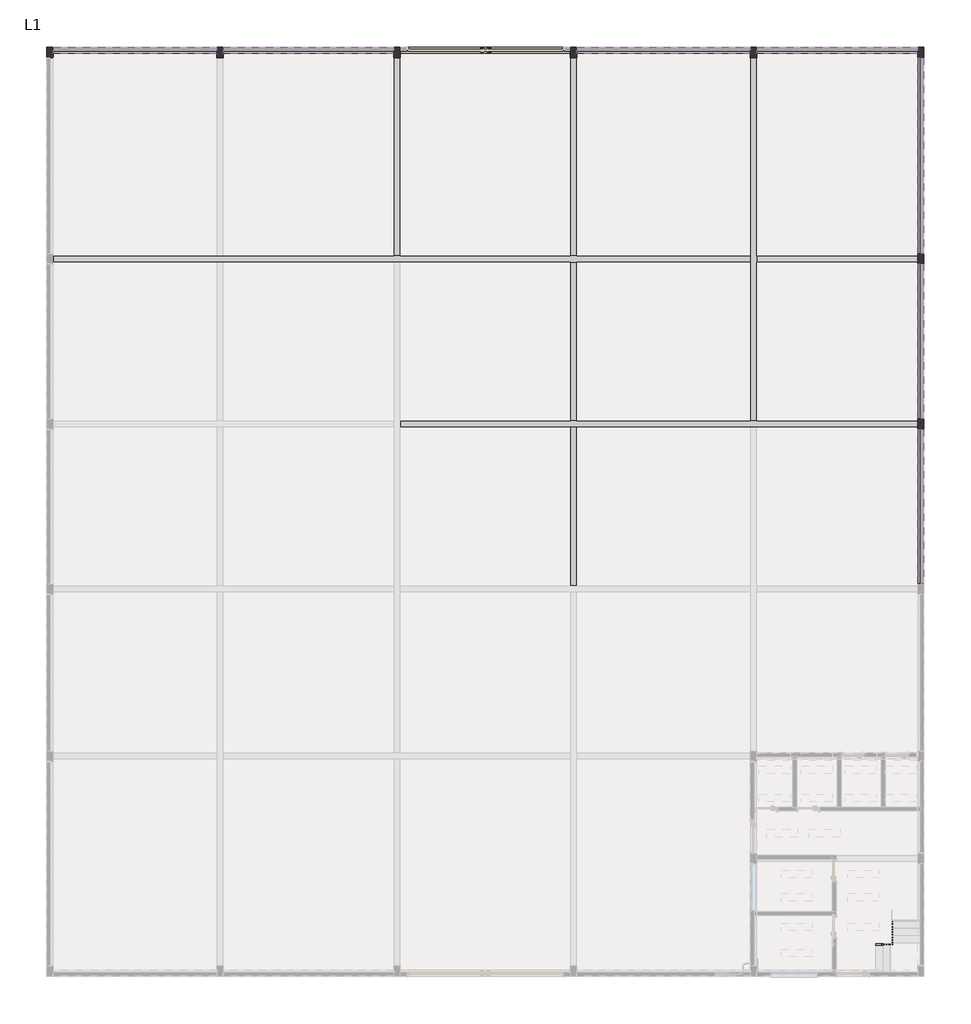
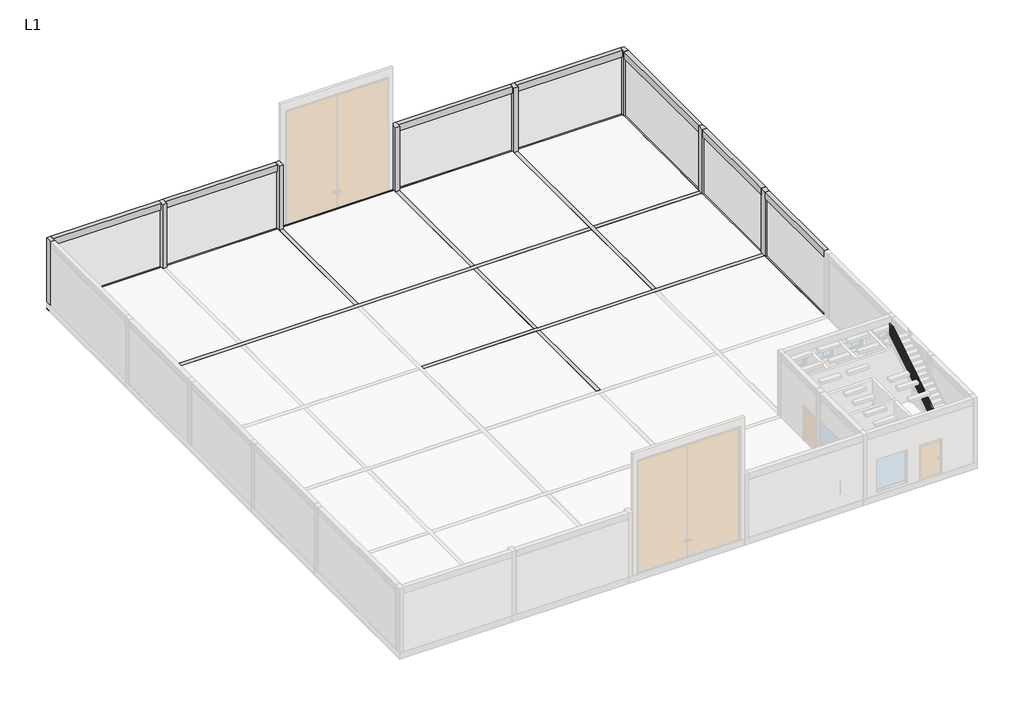
# One storey, part 3 of 4: 23 beams, 8 columns, 1 railing.
"""IFC4 building model written with IfcOpenShell, lengths in millimetres."""

from ifc_helpers import new_model, si_unit, frame, origin, place, context, project, spatial, polyline, outline, extrude, faceted_brep, element, save

model = new_model("IFC4")

# Units and contexts
model_context = context("Model", 3, world=origin())
ifc_project = project(units=[si_unit("LENGTHUNIT", "METRE", prefix="MILLI")], contexts=[model_context])

# Site, building, storey
site = spatial("IfcSite", under=ifc_project)
building = spatial("IfcBuilding", under=site)
storey = spatial("IfcBuildingStorey", under=building, Name="L1", Elevation=0.0)

# Beams
placement = place(None, origin())
element("IfcBeam", 1, ObjectType="M_Hormigón-Viga rectangular : 250 x 400mm", at=placement, inside=storey, context=model_context, shape_type="Brep", body=[
    faceted_brep([(10275.0, 18000.0, 0.0), (10275.0, 17750.0, 0.0), (10525.0, 17750.0, 0.0), (16750.0, 17750.0, 0.0), (17000.0, 17750.0, 0.0), (17000.0, 18000.0, 0.0), (10275.0, 18000.0, -400.0), (17000.0, 18000.0, -400.0), (10275.0, 17750.0, -400.0), (17000.0, 17750.0, -400.0), (16750.0, 17750.0, -400.0), (10525.0, 17750.0, -400.0)], [[[0, 1, 2, 3, 4, 5]], [[6, 0, 5, 7]], [[8, 6, 7, 9, 10, 11]], [[1, 8, 11, 10, 9, 4, 3, 2]], [[1, 0, 6, 8]], [[5, 4, 9, 7]]]),
])
element("IfcBeam", 2, ObjectType="M_Hormigón-Viga rectangular : 250 x 400mm", at=placement, inside=storey, context=model_context, shape_type="Brep", body=[
    faceted_brep([(3300.0, 18000.0, 0.0), (3300.0, 17750.0, 0.0), (3550.0, 17750.0, 0.0), (10275.0, 17750.0, 0.0), (10275.0, 18000.0, 0.0), (3300.0, 18000.0, -400.0), (10275.0, 18000.0, -400.0), (3300.0, 17750.0, -400.0), (10275.0, 17750.0, -400.0), (3550.0, 17750.0, -400.0), (10275.0, 17750.0, -350.0)], [[[0, 1, 2, 3, 4]], [[5, 0, 4, 6]], [[7, 5, 6, 8, 9]], [[1, 7, 9, 8, 10, 3, 2]], [[1, 0, 5, 7]], [[4, 3, 10, 8, 6]]]),
])
element("IfcBeam", 3, ObjectType="M_Hormigón-Viga rectangular : 250 x 400mm", at=placement, inside=storey, context=model_context, shape_type="Brep", body=[
    faceted_brep([(-3550.0, 18000.0, 0.0), (-3550.0, 17750.0, 0.0), (-3300.0, 17750.0, 0.0), (3300.0, 17750.0, 0.0), (3300.0, 18000.0, 0.0), (-3550.0, 18000.0, -400.0), (3300.0, 18000.0, -400.0), (-3550.0, 17750.0, -400.0), (3300.0, 17750.0, -400.0), (-3300.0, 17750.0, -400.0), (3300.0, 17750.0, -350.0)], [[[0, 1, 2, 3, 4]], [[5, 0, 4, 6]], [[7, 5, 6, 8, 9]], [[1, 7, 9, 8, 10, 3, 2]], [[1, 0, 5, 7]], [[4, 3, 10, 8, 6]]]),
])
element("IfcBeam", 4, ObjectType="M_Hormigón-Viga rectangular : 250 x 400mm", at=placement, inside=storey, context=model_context, shape_type="Brep", body=[
    faceted_brep([(-10400.0, 18000.0, 0.0), (-10400.0, 17750.0, 0.0), (-10150.0, 17750.0, 0.0), (-3550.0, 17750.0, 0.0), (-3550.0, 18000.0, 0.0), (-10400.0, 18000.0, -400.0), (-3550.0, 18000.0, -400.0), (-10400.0, 17750.0, -400.0), (-3550.0, 17750.0, -400.0), (-10150.0, 17750.0, -400.0), (-3550.0, 17750.0, -350.0)], [[[0, 1, 2, 3, 4]], [[5, 0, 4, 6]], [[7, 5, 6, 8, 9]], [[1, 7, 9, 8, 10, 3, 2]], [[1, 0, 5, 7]], [[4, 3, 10, 8, 6]]]),
])
element("IfcBeam", 5, ObjectType="M_Hormigón-Viga rectangular : 250 x 400mm", at=placement, inside=storey, context=model_context, shape_type="Brep", body=[
    faceted_brep([(-17000.0, 18000.0, 0.0), (-17000.0, 17750.0, 0.0), (-16750.0, 17750.0, 0.0), (-10400.0, 17750.0, 0.0), (-10400.0, 18000.0, 0.0), (-16750.0, 18000.0, 0.0), (-17000.0, 18000.0, -400.0), (-17000.0, 18000.0, -350.0), (-10400.0, 18000.0, -400.0), (-17000.0, 17750.0, -400.0), (-10400.0, 17750.0, -400.0), (-16750.0, 17750.0, -400.0), (-10400.0, 17750.0, -350.0)], [[[0, 1, 2, 3, 4, 5]], [[6, 7, 0, 5, 4, 8]], [[9, 6, 8, 10, 11]], [[1, 9, 11, 10, 12, 3, 2]], [[1, 0, 7, 6, 9]], [[4, 3, 12, 10, 8]]]),
])
element("IfcBeam", 6, ObjectType="M_Hormigón-Viga rectangular : 250 x 400mm", at=placement, inside=storey, context=model_context, shape_type="Brep", body=[
    faceted_brep([(17000.0, 9675.0, 0.0), (17000.0, 9925.0, 0.0), (16750.0, 9925.0, 0.0), (10525.0, 9925.0, 0.0), (10525.0, 9675.0, 0.0), (16750.0, 9675.0, 0.0), (17000.0, 9925.0, -400.0), (16750.0, 9925.0, -400.0), (10525.0, 9925.0, -400.0), (10525.0, 9925.0, -350.0), (17000.0, 9675.0, -400.0), (16750.0, 9675.0, -400.0), (10525.0, 9675.0, -400.0), (10525.0, 9675.0, -350.0)], [[[0, 1, 2, 3, 4, 5]], [[1, 6, 7, 8, 9, 3, 2]], [[6, 10, 11, 12, 8, 7]], [[10, 0, 5, 4, 13, 12, 11]], [[1, 0, 10, 6]], [[4, 3, 9, 8, 12, 13]]]),
])
element("IfcBeam", 7, ObjectType="M_Hormigón-Viga rectangular : 250 x 400mm", at=placement, inside=storey, context=model_context, shape_type="Brep", body=[
    faceted_brep([(17000.0, 3275.0, 0.0), (17000.0, 3525.0, 0.0), (16750.0, 3525.0, 0.0), (10525.0, 3525.0, 0.0), (10275.0, 3525.0, 0.0), (3550.0, 3525.0, 0.0), (3300.0, 3525.0, 0.0), (-3300.0, 3525.0, 0.0), (-3300.0, 3275.0, 0.0), (3300.0, 3275.0, 0.0), (3550.0, 3275.0, 0.0), (10275.0, 3275.0, 0.0), (10525.0, 3275.0, 0.0), (16750.0, 3275.0, 0.0), (17000.0, 3525.0, -400.0), (16750.0, 3525.0, -400.0), (10525.0, 3525.0, -400.0), (10275.0, 3525.0, -400.0), (3550.0, 3525.0, -400.0), (3300.0, 3525.0, -400.0), (-3300.0, 3525.0, -400.0), (-3300.0, 3525.0, -350.0), (17000.0, 3275.0, -400.0), (16750.0, 3275.0, -400.0), (10525.0, 3275.0, -400.0), (10275.0, 3275.0, -400.0), (3550.0, 3275.0, -400.0), (3300.0, 3275.0, -400.0), (-3300.0, 3275.0, -400.0), (-3300.0, 3275.0, -350.0)], [[[0, 1, 2, 3, 4, 5, 6, 7, 8, 9, 10, 11, 12, 13]], [[1, 14, 15, 16, 17, 18, 19, 20, 21, 7, 6, 5, 4, 3, 2]], [[14, 22, 23, 24, 25, 26, 27, 28, 20, 19, 18, 17, 16, 15]], [[22, 0, 13, 12, 11, 10, 9, 8, 29, 28, 27, 26, 25, 24, 23]], [[1, 0, 22, 14]], [[8, 7, 21, 20, 28, 29]]]),
])
element("IfcBeam", 8, ObjectType="M_Hormigón-Viga rectangular : 250 x 400mm", at=placement, inside=storey, context=model_context, shape_type="Brep", body=[
    faceted_brep([(17000.0, 3275.0, 0.0), (16750.0, 3275.0, 0.0), (16750.0, 3200.0, 0.0), (16750.0, -2800.0, 0.0), (16750.0, -2875.0, 0.0), (17000.0, -2875.0, 0.0), (17000.0, -2800.0, 0.0), (17000.0, 3200.0, 0.0), (17000.0, 3275.0, -400.0), (17000.0, -2875.0, -400.0), (16750.0, 3275.0, -400.0), (16750.0, -2875.0, -400.0), (16750.0, 3275.0, -350.0), (16750.0, -2875.0, -350.0)], [[[0, 1, 2, 3, 4, 5, 6, 7]], [[8, 0, 7, 6, 5, 9]], [[10, 8, 9, 11]], [[1, 12, 10, 11, 13, 4, 3, 2]], [[1, 0, 8, 10, 12]], [[5, 4, 13, 11, 9]]]),
])
element("IfcBeam", 9, ObjectType="M_Hormigón-Viga rectangular : 250 x 400mm", at=placement, inside=storey, context=model_context, shape_type="Brep", body=[
    faceted_brep([(17000.0, 9675.0, 0.0), (16750.0, 9675.0, 0.0), (16750.0, 9600.0, 0.0), (16750.0, 3600.0, 0.0), (16750.0, 3525.0, 0.0), (17000.0, 3525.0, 0.0), (17000.0, 3600.0, 0.0), (17000.0, 9600.0, 0.0), (17000.0, 9675.0, -400.0), (17000.0, 3525.0, -400.0), (16750.0, 9675.0, -400.0), (16750.0, 3525.0, -400.0), (16750.0, 9675.0, -350.0), (16750.0, 3525.0, -350.0)], [[[0, 1, 2, 3, 4, 5, 6, 7]], [[8, 0, 7, 6, 5, 9]], [[10, 8, 9, 11]], [[1, 12, 10, 11, 13, 4, 3, 2]], [[1, 0, 8, 10, 12]], [[5, 4, 13, 11, 9]]]),
])
element("IfcBeam", 10, ObjectType="M_Hormigón-Viga rectangular : 250 x 400mm", at=placement, inside=storey, context=model_context, shape_type="Brep", body=[
    faceted_brep([(16750.0, 9925.0, 0.0), (17000.0, 9925.0, 0.0), (17000.0, 10000.0, 0.0), (17000.0, 17600.0, 0.0), (17000.0, 17750.0, 0.0), (16750.0, 17750.0, 0.0), (16750.0, 17600.0, 0.0), (16750.0, 10000.0, 0.0), (17000.0, 9925.0, -400.0), (17000.0, 17750.0, -400.0), (16750.0, 9925.0, -400.0), (16750.0, 17750.0, -400.0), (16750.0, 9925.0, -350.0), (16750.0, 17750.0, -350.0)], [[[0, 1, 2, 3, 4, 5, 6, 7]], [[1, 8, 9, 4, 3, 2]], [[8, 10, 11, 9]], [[10, 12, 0, 7, 6, 5, 13, 11]], [[1, 0, 12, 10, 8]], [[5, 4, 9, 11, 13]]]),
])
element("IfcBeam", 11, ObjectType="M_Hormigón-Viga rectangular : 250 x 400mm", at=placement, inside=storey, context=model_context, shape_type="Brep", body=[
    faceted_brep([(-3300.0, 17750.0, 0.0), (-3550.0, 17750.0, 0.0), (-3550.0, 9925.0, 0.0), (-3300.0, 9925.0, 0.0), (-3300.0, 17750.0, -400.0), (-3300.0, 17750.0, -350.0), (-3300.0, 9925.0, -350.0), (-3300.0, 9925.0, -400.0), (-3550.0, 17750.0, -400.0), (-3550.0, 9925.0, -400.0), (-3550.0, 17750.0, -350.0), (-3550.0, 9925.0, -350.0)], [[[0, 1, 2, 3]], [[4, 5, 0, 3, 6, 7]], [[8, 4, 7, 9]], [[1, 10, 8, 9, 11, 2]], [[1, 0, 5, 4, 8, 10]], [[3, 2, 11, 9, 7, 6]]]),
])
element("IfcBeam", 12, ObjectType="M_Hormigón-Viga rectangular : 250 x 400mm", at=placement, inside=storey, context=model_context, shape_type="Brep", body=[
    faceted_brep([(3550.0, 17750.0, 0.0), (3300.0, 17750.0, 0.0), (3300.0, 9925.0, 0.0), (3550.0, 9925.0, 0.0), (3550.0, 17750.0, -400.0), (3550.0, 17750.0, -350.0), (3550.0, 9925.0, -350.0), (3550.0, 9925.0, -400.0), (3300.0, 17750.0, -400.0), (3300.0, 9925.0, -400.0), (3300.0, 17750.0, -350.0), (3300.0, 9925.0, -350.0)], [[[0, 1, 2, 3]], [[4, 5, 0, 3, 6, 7]], [[8, 4, 7, 9]], [[1, 10, 8, 9, 11, 2]], [[1, 0, 5, 4, 8, 10]], [[3, 2, 11, 9, 7, 6]]]),
])
element("IfcBeam", 13, ObjectType="M_Hormigón-Viga rectangular : 250 x 400mm", at=placement, inside=storey, context=model_context, shape_type="Brep", body=[
    faceted_brep([(-16750.0, 9925.0, 0.0), (-16750.0, 9675.0, 0.0), (-10400.0, 9675.0, 0.0), (-10150.0, 9675.0, 0.0), (-3550.0, 9675.0, 0.0), (-3300.0, 9675.0, 0.0), (3300.0, 9675.0, 0.0), (3550.0, 9675.0, 0.0), (10275.0, 9675.0, 0.0), (10275.0, 9925.0, 0.0), (3550.0, 9925.0, 0.0), (3300.0, 9925.0, 0.0), (-3300.0, 9925.0, 0.0), (-3550.0, 9925.0, 0.0), (-10150.0, 9925.0, 0.0), (-10400.0, 9925.0, 0.0), (-16750.0, 9925.0, -400.0), (-16750.0, 9925.0, -350.0), (10275.0, 9925.0, -350.0), (10275.0, 9925.0, -400.0), (3550.0, 9925.0, -400.0), (3300.0, 9925.0, -400.0), (-3300.0, 9925.0, -400.0), (-3550.0, 9925.0, -400.0), (-10150.0, 9925.0, -400.0), (-10400.0, 9925.0, -400.0), (-16750.0, 9675.0, -400.0), (10275.0, 9675.0, -400.0), (3550.0, 9675.0, -400.0), (3300.0, 9675.0, -400.0), (-3300.0, 9675.0, -400.0), (-3550.0, 9675.0, -400.0), (-10150.0, 9675.0, -400.0), (-10400.0, 9675.0, -400.0), (-16750.0, 9675.0, -350.0), (10275.0, 9675.0, -350.0)], [[[0, 1, 2, 3, 4, 5, 6, 7, 8, 9, 10, 11, 12, 13, 14, 15]], [[16, 17, 0, 15, 14, 13, 12, 11, 10, 9, 18, 19, 20, 21, 22, 23, 24, 25]], [[26, 16, 25, 24, 23, 22, 21, 20, 19, 27, 28, 29, 30, 31, 32, 33]], [[1, 34, 26, 33, 32, 31, 30, 29, 28, 27, 35, 8, 7, 6, 5, 4, 3, 2]], [[1, 0, 17, 16, 26, 34]], [[9, 8, 35, 27, 19, 18]]]),
])
element("IfcBeam", 14, ObjectType="M_Hormigón-Viga rectangular : 250 x 400mm", at=placement, inside=storey, context=model_context, shape_type="Brep", body=[
    faceted_brep([(3550.0, 9675.0, 0.0), (3300.0, 9675.0, 0.0), (3300.0, 3525.0, 0.0), (3550.0, 3525.0, 0.0), (3550.0, 9675.0, -400.0), (3550.0, 9675.0, -350.0), (3550.0, 3525.0, -350.0), (3550.0, 3525.0, -400.0), (3300.0, 9675.0, -400.0), (3300.0, 3525.0, -400.0), (3300.0, 9675.0, -350.0), (3300.0, 3525.0, -350.0)], [[[0, 1, 2, 3]], [[4, 5, 0, 3, 6, 7]], [[8, 4, 7, 9]], [[1, 10, 8, 9, 11, 2]], [[1, 0, 5, 4, 8, 10]], [[3, 2, 11, 9, 7, 6]]]),
])
element("IfcBeam", 15, ObjectType="M_Hormigón-Viga rectangular : 250 x 400mm", at=placement, inside=storey, context=model_context, shape_type="Brep", body=[
    faceted_brep([(10525.0, 17750.0, 0.0), (10275.0, 17750.0, 0.0), (10275.0, 9925.0, 0.0), (10275.0, 9675.0, 0.0), (10275.0, 3525.0, 0.0), (10525.0, 3525.0, 0.0), (10525.0, 9675.0, 0.0), (10525.0, 9925.0, 0.0), (10525.0, 17750.0, -400.0), (10525.0, 17750.0, -350.0), (10525.0, 3525.0, -350.0), (10525.0, 3525.0, -400.0), (10525.0, 9675.0, -400.0), (10525.0, 9925.0, -400.0), (10275.0, 17750.0, -400.0), (10275.0, 3525.0, -400.0), (10275.0, 9675.0, -400.0), (10275.0, 9925.0, -400.0), (10275.0, 17750.0, -350.0), (10275.0, 3525.0, -350.0)], [[[0, 1, 2, 3, 4, 5, 6, 7]], [[8, 9, 0, 7, 6, 5, 10, 11, 12, 13]], [[14, 8, 13, 12, 11, 15, 16, 17]], [[1, 18, 14, 17, 16, 15, 19, 4, 3, 2]], [[1, 0, 9, 8, 14, 18]], [[5, 4, 19, 15, 11, 10]]]),
])
element("IfcBeam", 16, ObjectType="M_Hormigón-Viga rectangular : 250 x 400mm", at=placement, inside=storey, context=model_context, shape_type="Brep", body=[
    faceted_brep([(3550.0, 3275.0, 0.0), (3300.0, 3275.0, 0.0), (3300.0, -2875.0, 0.0), (3550.0, -2875.0, 0.0), (3550.0, 3275.0, -400.0), (3550.0, 3275.0, -350.0), (3550.0, -2875.0, -350.0), (3550.0, -2875.0, -400.0), (3300.0, 3275.0, -400.0), (3300.0, -2875.0, -400.0), (3300.0, 3275.0, -350.0), (3300.0, -2875.0, -350.0)], [[[0, 1, 2, 3]], [[4, 5, 0, 3, 6, 7]], [[8, 4, 7, 9]], [[1, 10, 8, 9, 11, 2]], [[1, 0, 5, 4, 8, 10]], [[3, 2, 11, 9, 7, 6]]]),
])
element("IfcBeam", 17, ObjectType="M_Hormigón-Viga rectangular : 250 x 400mm", at=placement, inside=storey, context=model_context, shape_type="SweptSolid", body=[
    extrude(outline(polyline([(10525.0, 17750.0), (10525.0, 18000.0), (16750.0, 18000.0), (16750.0, 17750.0), (10525.0, 17750.0)])), frame((0.0, 0.0, 3600.0), z_axis=(0.0, 0.0, 1.0), x_axis=(1.0, 0.0, 0.0)), (0.0, 0.0, 1.0), 400.0),
])
element("IfcBeam", 18, ObjectType="M_Hormigón-Viga rectangular : 250 x 400mm", at=placement, inside=storey, context=model_context, shape_type="SweptSolid", body=[
    extrude(outline(polyline([(3550.0, 17750.0), (3550.0, 18000.0), (10275.0, 18000.0), (10275.0, 17750.0), (3550.0, 17750.0)])), frame((0.0, 0.0, 3600.0), z_axis=(0.0, 0.0, 1.0), x_axis=(1.0, 0.0, 0.0)), (0.0, 0.0, 1.0), 400.0),
])
element("IfcBeam", 19, ObjectType="M_Hormigón-Viga rectangular : 250 x 400mm", at=placement, inside=storey, context=model_context, shape_type="SweptSolid", body=[
    extrude(outline(polyline([(-3550.0, 18000.0), (-3550.0, 17750.0), (-10150.0, 17750.0), (-10150.0, 18000.0), (-3550.0, 18000.0)])), frame((0.0, 0.0, 3600.0), z_axis=(0.0, 0.0, 1.0), x_axis=(1.0, 0.0, 0.0)), (0.0, 0.0, 1.0), 400.0),
])
element("IfcBeam", 20, ObjectType="M_Hormigón-Viga rectangular : 250 x 400mm", at=placement, inside=storey, context=model_context, shape_type="SweptSolid", body=[
    extrude(outline(polyline([(-16750.0, 17750.0), (-16750.0, 18000.0), (-10400.0, 18000.0), (-10400.0, 17750.0), (-16750.0, 17750.0)])), frame((0.0, 0.0, 3600.0), z_axis=(0.0, 0.0, 1.0), x_axis=(1.0, 0.0, 0.0)), (0.0, 0.0, 1.0), 400.0),
])
element("IfcBeam", 21, ObjectType="M_Hormigón-Viga rectangular : 250 x 400mm", at=placement, inside=storey, context=model_context, shape_type="SweptSolid", body=[
    extrude(outline(polyline([(16750.0, 3200.0), (17000.0, 3200.0), (17000.0, -2800.0), (16750.0, -2800.0), (16750.0, 3200.0)])), frame((0.0, 0.0, 3600.0), z_axis=(0.0, 0.0, 1.0), x_axis=(1.0, 0.0, 0.0)), (0.0, 0.0, 1.0), 400.0),
])
element("IfcBeam", 22, ObjectType="M_Hormigón-Viga rectangular : 250 x 400mm", at=placement, inside=storey, context=model_context, shape_type="SweptSolid", body=[
    extrude(outline(polyline([(16750.0, 9600.0), (17000.0, 9600.0), (17000.0, 3600.0), (16750.0, 3600.0), (16750.0, 9600.0)])), frame((0.0, 0.0, 3600.0), z_axis=(0.0, 0.0, 1.0), x_axis=(1.0, 0.0, 0.0)), (0.0, 0.0, 1.0), 400.0),
])
element("IfcBeam", 23, ObjectType="M_Hormigón-Viga rectangular : 250 x 400mm", at=placement, inside=storey, context=model_context, shape_type="SweptSolid", body=[
    extrude(outline(polyline([(16750.0, 17600.0), (17000.0, 17600.0), (17000.0, 10000.0), (16750.0, 10000.0), (16750.0, 17600.0)])), frame((0.0, 0.0, 3600.0), z_axis=(0.0, 0.0, 1.0), x_axis=(1.0, 0.0, 0.0)), (0.0, 0.0, 1.0), 400.0),
])

# Columns
element("IfcColumn", 24, ObjectType="M_Hormigón-Rectangular-Pilar : 250 x 400mm", at=placement, inside=storey, context=model_context, shape_type="Brep", body=[
    faceted_brep([(-17000.0, 17600.0, 0.0), (-17000.0, 17750.0, 0.0), (-17000.0, 18000.0, 0.0), (-16750.0, 18000.0, 0.0), (-16750.0, 17750.0, 0.0), (-16750.0, 17600.0, 0.0), (-17000.0, 17600.0, 4000.0), (-17000.0, 18000.0, 4000.0), (-16750.0, 18000.0, 4000.0), (-16750.0, 17600.0, 4000.0)], [[[0, 1, 2, 3, 4, 5]], [[6, 7, 2, 1, 0]], [[7, 8, 3, 2]], [[8, 9, 5, 4, 3]], [[9, 6, 0, 5]], [[6, 9, 8, 7]]]),
])
element("IfcColumn", 25, ObjectType="M_Hormigón-Rectangular-Pilar : 250 x 400mm", at=placement, inside=storey, context=model_context, shape_type="Brep", body=[
    faceted_brep([(-3550.0, 17600.0, 0.0), (-3550.0, 17750.0, 0.0), (-3550.0, 18000.0, 0.0), (-3300.0, 18000.0, 0.0), (-3300.0, 17750.0, 0.0), (-3300.0, 17600.0, 0.0), (-3550.0, 17600.0, 4000.0), (-3550.0, 18000.0, 4000.0), (-3300.0, 18000.0, 4000.0), (-3300.0, 17600.0, 4000.0)], [[[0, 1, 2, 3, 4, 5]], [[6, 7, 2, 1, 0]], [[7, 8, 3, 2]], [[8, 9, 5, 4, 3]], [[9, 6, 0, 5]], [[6, 9, 8, 7]]]),
])
element("IfcColumn", 26, ObjectType="M_Hormigón-Rectangular-Pilar : 250 x 400mm", at=placement, inside=storey, context=model_context, shape_type="Brep", body=[
    faceted_brep([(3300.0, 17600.0, 0.0), (3300.0, 17750.0, 0.0), (3300.0, 18000.0, 0.0), (3550.0, 18000.0, 0.0), (3550.0, 17750.0, 0.0), (3550.0, 17600.0, 0.0), (3300.0, 17600.0, 4000.0), (3300.0, 18000.0, 4000.0), (3550.0, 18000.0, 4000.0), (3550.0, 17600.0, 4000.0)], [[[0, 1, 2, 3, 4, 5]], [[6, 7, 2, 1, 0]], [[7, 8, 3, 2]], [[8, 9, 5, 4, 3]], [[9, 6, 0, 5]], [[6, 9, 8, 7]]]),
])
element("IfcColumn", 27, ObjectType="M_Hormigón-Rectangular-Pilar : 250 x 400mm", at=placement, inside=storey, context=model_context, shape_type="Brep", body=[
    faceted_brep([(10275.0, 17600.0, 0.0), (10275.0, 17750.0, 0.0), (10275.0, 18000.0, 0.0), (10525.0, 18000.0, 0.0), (10525.0, 17750.0, 0.0), (10525.0, 17600.0, 0.0), (10275.0, 17600.0, 4000.0), (10275.0, 18000.0, 4000.0), (10525.0, 18000.0, 4000.0), (10525.0, 17600.0, 4000.0)], [[[0, 1, 2, 3, 4, 5]], [[6, 7, 2, 1, 0]], [[7, 8, 3, 2]], [[8, 9, 5, 4, 3]], [[9, 6, 0, 5]], [[6, 9, 8, 7]]]),
])
element("IfcColumn", 28, ObjectType="M_Hormigón-Rectangular-Pilar : 250 x 400mm", at=placement, inside=storey, context=model_context, shape_type="Brep", body=[
    faceted_brep([(16750.0, 17600.0, 0.0), (16750.0, 17750.0, 0.0), (16750.0, 18000.0, 0.0), (17000.0, 18000.0, 0.0), (17000.0, 17750.0, 0.0), (17000.0, 17600.0, 0.0), (16750.0, 17600.0, 4000.0), (16750.0, 18000.0, 4000.0), (17000.0, 18000.0, 4000.0), (17000.0, 17600.0, 4000.0)], [[[0, 1, 2, 3, 4, 5]], [[6, 7, 2, 1, 0]], [[7, 8, 3, 2]], [[8, 9, 5, 4, 3]], [[9, 6, 0, 5]], [[6, 9, 8, 7]]]),
])
element("IfcColumn", 29, ObjectType="M_Hormigón-Rectangular-Pilar : 250 x 400mm", at=placement, inside=storey, context=model_context, shape_type="Brep", body=[
    faceted_brep([(-10400.0, 17600.0, 0.0), (-10400.0, 17750.0, 0.0), (-10400.0, 18000.0, 0.0), (-10150.0, 18000.0, 0.0), (-10150.0, 17750.0, 0.0), (-10150.0, 17600.0, 0.0), (-10400.0, 17600.0, 4000.0), (-10400.0, 18000.0, 4000.0), (-10150.0, 18000.0, 4000.0), (-10150.0, 17600.0, 4000.0)], [[[0, 1, 2, 3, 4, 5]], [[6, 7, 2, 1, 0]], [[7, 8, 3, 2]], [[8, 9, 5, 4, 3]], [[9, 6, 0, 5]], [[6, 9, 8, 7]]]),
])
element("IfcColumn", 30, ObjectType="M_Hormigón-Rectangular-Pilar : 250 x 400mm", at=placement, inside=storey, context=model_context, shape_type="Brep", body=[
    faceted_brep([(16750.0, 9600.0, 0.0), (16750.0, 9675.0, 0.0), (16750.0, 9925.0, 0.0), (16750.0, 10000.0, 0.0), (17000.0, 10000.0, 0.0), (17000.0, 9925.0, 0.0), (17000.0, 9675.0, 0.0), (17000.0, 9600.0, 0.0), (16750.0, 9600.0, 4000.0), (16750.0, 10000.0, 4000.0), (17000.0, 10000.0, 4000.0), (17000.0, 9600.0, 4000.0)], [[[0, 1, 2, 3, 4, 5, 6, 7]], [[8, 9, 3, 2, 1, 0]], [[9, 10, 4, 3]], [[10, 11, 7, 6, 5, 4]], [[11, 8, 0, 7]], [[8, 11, 10, 9]]]),
])
element("IfcColumn", 31, ObjectType="M_Hormigón-Rectangular-Pilar : 250 x 400mm", at=placement, inside=storey, context=model_context, shape_type="Brep", body=[
    faceted_brep([(16750.0, 3200.0, 0.0), (16750.0, 3275.0, 0.0), (16750.0, 3525.0, 0.0), (16750.0, 3600.0, 0.0), (17000.0, 3600.0, 0.0), (17000.0, 3525.0, 0.0), (17000.0, 3275.0, 0.0), (17000.0, 3200.0, 0.0), (16750.0, 3200.0, 4000.0), (16750.0, 3600.0, 4000.0), (17000.0, 3600.0, 4000.0), (17000.0, 3200.0, 4000.0)], [[[0, 1, 2, 3, 4, 5, 6, 7]], [[8, 9, 3, 2, 1, 0]], [[9, 10, 4, 3]], [[10, 11, 7, 6, 5, 4]], [[11, 8, 0, 7]], [[8, 11, 10, 9]]]),
])

# Railing
element("IfcRailing", 32, ObjectType="Pasamanos - Rectangular", at=placement, inside=storey, context=model_context, shape_type="SolidModel", body=[
    faceted_brep([(15137.5726879, -16747.8618478, 1073.9130435), (15137.5726879, -16747.8618478, 1014.753434), (15137.5726879, -16797.8618478, 1014.753434), (15137.5726879, -16797.8618478, 1073.9130435), (15687.5726879, -16747.8618478, 1421.7391304), (15702.0563204, -16747.8618478, 1371.7391304), (15702.0563204, -16797.8618478, 1371.7391304), (15687.5726879, -16797.8618478, 1421.7391304), (15797.9726879, -16747.8618478, 1421.7391304), (15797.9726879, -16797.8618478, 1421.7391304), (15797.9726879, -16797.8618478, 1371.7391304), (15797.9726879, -16747.8618478, 1371.7391304)], [[[0, 1, 2, 3]], [[1, 0, 4, 5]], [[2, 1, 5, 6]], [[3, 2, 6, 7]], [[0, 3, 7, 4]], [[8, 9, 10, 11]], [[5, 4, 8, 11]], [[6, 5, 11, 10]], [[7, 6, 10, 9]], [[4, 7, 9, 8]]]),
    faceted_brep([(15747.9726879, -16747.8618478, 1480.4200194), (15747.9726879, -16747.8618478, 1352.8512657), (15797.9726879, -16747.8618478, 1352.8512657), (15797.9726879, -16747.8618478, 1480.4200194), (15747.9726879, -16698.7691378, 1595.6521739), (15747.9726879, -16658.8763415, 1561.7212103), (15797.9726879, -16658.8763415, 1561.7212103), (15797.9726879, -16698.7691378, 1595.6521739), (15747.9726879, -11473.7691378, 4900.0), (15747.9726879, -11459.2855053, 4850.0), (15797.9726879, -11459.2855053, 4850.0), (15797.9726879, -11473.7691378, 4900.0), (15747.9726879, -11198.7691378, 4900.0), (15797.9726879, -11198.7691378, 4900.0), (15797.9726879, -11198.7691378, 4850.0), (15747.9726879, -11198.7691378, 4850.0)], [[[0, 1, 2, 3]], [[1, 0, 4, 5]], [[2, 1, 5, 6]], [[3, 2, 6, 7]], [[0, 3, 7, 4]], [[5, 4, 8, 9]], [[6, 5, 9, 10]], [[7, 6, 10, 11]], [[4, 7, 11, 8]], [[12, 13, 14, 15]], [[9, 8, 12, 15]], [[10, 9, 15, 14]], [[11, 10, 14, 13]], [[8, 11, 13, 12]]]),
    extrude(outline(polyline([(15762.9726879, -11222.3691378), (15762.9726879, -11202.3691378), (15782.9726879, -11202.3691378), (15782.9726879, -11222.3691378), (15762.9726879, -11222.3691378)])), frame((0.0, 0.0, 4000.0), z_axis=(0.0, 0.0, 1.0), x_axis=(1.0, 0.0, 0.0)), (0.0, 0.0, 1.0), 850.0),
    extrude(outline(polyline([(15762.9726879, -11323.9691378), (15762.9726879, -11303.9691378), (15782.9726879, -11303.9691378), (15782.9726879, -11323.9691378), (15762.9726879, -11323.9691378)])), frame((0.0, 0.0, 4000.0), z_axis=(0.0, 0.0, 1.0), x_axis=(1.0, 0.0, 0.0)), (0.0, 0.0, 1.0), 850.0),
    extrude(outline(polyline([(15762.9726879, -11425.5691378), (15762.9726879, -11405.5691378), (15782.9726879, -11405.5691378), (15782.9726879, -11425.5691378), (15762.9726879, -11425.5691378)])), frame((0.0, 0.0, 4000.0), z_axis=(0.0, 0.0, 1.0), x_axis=(1.0, 0.0, 0.0)), (0.0, 0.0, 1.0), 850.0),
    extrude(outline(polyline([(-11527.1691378, 4807.0696395), (-11507.1691378, 4819.7178609), (-11507.1691378, 3826.0869565), (-11527.1691378, 3826.0869565), (-11527.1691378, 4807.0696395)])), frame((15762.9726879, 0.0, 0.0), z_axis=(1.0, 0.0, 0.0), x_axis=(0.0, 1.0, 0.0)), (0.0, 0.0, 1.0), 20.0),
    extrude(outline(polyline([(-11628.7691378, 4742.8166751), (-11608.7691378, 4755.4648964), (-11608.7691378, 3826.0869565), (-11628.7691378, 3826.0869565), (-11628.7691378, 4742.8166751)])), frame((15762.9726879, 0.0, 0.0), z_axis=(1.0, 0.0, 0.0), x_axis=(0.0, 1.0, 0.0)), (0.0, 0.0, 1.0), 20.0),
    extrude(outline(polyline([(-11730.3691378, 4678.5637107), (-11710.3691378, 4691.211932), (-11710.3691378, 3826.0869565), (-11730.3691378, 3826.0869565), (-11730.3691378, 4678.5637107)])), frame((15762.9726879, 0.0, 0.0), z_axis=(1.0, 0.0, 0.0), x_axis=(0.0, 1.0, 0.0)), (0.0, 0.0, 1.0), 20.0),
    extrude(outline(polyline([(-11831.9691378, 4614.3107462), (-11811.9691378, 4626.9589676), (-11811.9691378, 3652.173913), (-11831.9691378, 3652.173913), (-11831.9691378, 4614.3107462)])), frame((15762.9726879, 0.0, 0.0), z_axis=(1.0, 0.0, 0.0), x_axis=(0.0, 1.0, 0.0)), (0.0, 0.0, 1.0), 20.0),
    extrude(outline(polyline([(-11933.5691378, 4550.0577818), (-11913.5691378, 4562.7060032), (-11913.5691378, 3652.173913), (-11933.5691378, 3652.173913), (-11933.5691378, 4550.0577818)])), frame((15762.9726879, 0.0, 0.0), z_axis=(1.0, 0.0, 0.0), x_axis=(0.0, 1.0, 0.0)), (0.0, 0.0, 1.0), 20.0),
    extrude(outline(polyline([(-12035.1691378, 4485.8048174), (-12015.1691378, 4498.4530387), (-12015.1691378, 3478.2608696), (-12035.1691378, 3478.2608696), (-12035.1691378, 4485.8048174)])), frame((15762.9726879, 0.0, 0.0), z_axis=(1.0, 0.0, 0.0), x_axis=(0.0, 1.0, 0.0)), (0.0, 0.0, 1.0), 20.0),
    extrude(outline(polyline([(-12136.7691378, 4421.551853), (-12116.7691378, 4434.2000743), (-12116.7691378, 3478.2608696), (-12136.7691378, 3478.2608696), (-12136.7691378, 4421.551853)])), frame((15762.9726879, 0.0, 0.0), z_axis=(1.0, 0.0, 0.0), x_axis=(0.0, 1.0, 0.0)), (0.0, 0.0, 1.0), 20.0),
    extrude(outline(polyline([(-12238.3691378, 4357.2988885), (-12218.3691378, 4369.9471099), (-12218.3691378, 3478.2608696), (-12238.3691378, 3478.2608696), (-12238.3691378, 4357.2988885)])), frame((15762.9726879, 0.0, 0.0), z_axis=(1.0, 0.0, 0.0), x_axis=(0.0, 1.0, 0.0)), (0.0, 0.0, 1.0), 20.0),
    extrude(outline(polyline([(-12339.9691378, 4293.0459241), (-12319.9691378, 4305.6941455), (-12319.9691378, 3304.3478261), (-12339.9691378, 3304.3478261), (-12339.9691378, 4293.0459241)])), frame((15762.9726879, 0.0, 0.0), z_axis=(1.0, 0.0, 0.0), x_axis=(0.0, 1.0, 0.0)), (0.0, 0.0, 1.0), 20.0),
    extrude(outline(polyline([(-12441.5691378, 4228.7929597), (-12421.5691378, 4241.441181), (-12421.5691378, 3304.3478261), (-12441.5691378, 3304.3478261), (-12441.5691378, 4228.7929597)])), frame((15762.9726879, 0.0, 0.0), z_axis=(1.0, 0.0, 0.0), x_axis=(0.0, 1.0, 0.0)), (0.0, 0.0, 1.0), 20.0),
    extrude(outline(polyline([(-12543.1691378, 4164.5399953), (-12523.1691378, 4177.1882166), (-12523.1691378, 3304.3478261), (-12543.1691378, 3304.3478261), (-12543.1691378, 4164.5399953)])), frame((15762.9726879, 0.0, 0.0), z_axis=(1.0, 0.0, 0.0), x_axis=(0.0, 1.0, 0.0)), (0.0, 0.0, 1.0), 20.0),
    extrude(outline(polyline([(-12644.7691378, 4100.2870308), (-12624.7691378, 4112.9352522), (-12624.7691378, 3130.4347826), (-12644.7691378, 3130.4347826), (-12644.7691378, 4100.2870308)])), frame((15762.9726879, 0.0, 0.0), z_axis=(1.0, 0.0, 0.0), x_axis=(0.0, 1.0, 0.0)), (0.0, 0.0, 1.0), 20.0),
    extrude(outline(polyline([(-12746.3691378, 4036.0340664), (-12726.3691378, 4048.6822877), (-12726.3691378, 3130.4347826), (-12746.3691378, 3130.4347826), (-12746.3691378, 4036.0340664)])), frame((15762.9726879, 0.0, 0.0), z_axis=(1.0, 0.0, 0.0), x_axis=(0.0, 1.0, 0.0)), (0.0, 0.0, 1.0), 20.0),
    extrude(outline(polyline([(-12847.9691378, 3971.781102), (-12827.9691378, 3984.4293233), (-12827.9691378, 3130.4347826), (-12847.9691378, 3130.4347826), (-12847.9691378, 3971.781102)])), frame((15762.9726879, 0.0, 0.0), z_axis=(1.0, 0.0, 0.0), x_axis=(0.0, 1.0, 0.0)), (0.0, 0.0, 1.0), 20.0),
    extrude(outline(polyline([(-12949.5691378, 3907.5281375), (-12929.5691378, 3920.1763589), (-12929.5691378, 2956.5217391), (-12949.5691378, 2956.5217391), (-12949.5691378, 3907.5281375)])), frame((15762.9726879, 0.0, 0.0), z_axis=(1.0, 0.0, 0.0), x_axis=(0.0, 1.0, 0.0)), (0.0, 0.0, 1.0), 20.0),
    extrude(outline(polyline([(-13051.1691378, 3843.2751731), (-13031.1691378, 3855.9233945), (-13031.1691378, 2956.5217391), (-13051.1691378, 2956.5217391), (-13051.1691378, 3843.2751731)])), frame((15762.9726879, 0.0, 0.0), z_axis=(1.0, 0.0, 0.0), x_axis=(0.0, 1.0, 0.0)), (0.0, 0.0, 1.0), 20.0),
    extrude(outline(polyline([(-13152.7691378, 3779.0222087), (-13132.7691378, 3791.67043), (-13132.7691378, 2782.6086957), (-13152.7691378, 2782.6086957), (-13152.7691378, 3779.0222087)])), frame((15762.9726879, 0.0, 0.0), z_axis=(1.0, 0.0, 0.0), x_axis=(0.0, 1.0, 0.0)), (0.0, 0.0, 1.0), 20.0),
    extrude(outline(polyline([(-13254.3691378, 3714.7692443), (-13234.3691378, 3727.4174656), (-13234.3691378, 2782.6086957), (-13254.3691378, 2782.6086957), (-13254.3691378, 3714.7692443)])), frame((15762.9726879, 0.0, 0.0), z_axis=(1.0, 0.0, 0.0), x_axis=(0.0, 1.0, 0.0)), (0.0, 0.0, 1.0), 20.0),
    extrude(outline(polyline([(-13355.9691378, 3650.5162798), (-13335.9691378, 3663.1645012), (-13335.9691378, 2782.6086957), (-13355.9691378, 2782.6086957), (-13355.9691378, 3650.5162798)])), frame((15762.9726879, 0.0, 0.0), z_axis=(1.0, 0.0, 0.0), x_axis=(0.0, 1.0, 0.0)), (0.0, 0.0, 1.0), 20.0),
    extrude(outline(polyline([(-13457.5691378, 3586.2633154), (-13437.5691378, 3598.9115368), (-13437.5691378, 2608.6956522), (-13457.5691378, 2608.6956522), (-13457.5691378, 3586.2633154)])), frame((15762.9726879, 0.0, 0.0), z_axis=(1.0, 0.0, 0.0), x_axis=(0.0, 1.0, 0.0)), (0.0, 0.0, 1.0), 20.0),
    extrude(outline(polyline([(-13559.1691378, 3522.010351), (-13539.1691378, 3534.6585723), (-13539.1691378, 2608.6956522), (-13559.1691378, 2608.6956522), (-13559.1691378, 3522.010351)])), frame((15762.9726879, 0.0, 0.0), z_axis=(1.0, 0.0, 0.0), x_axis=(0.0, 1.0, 0.0)), (0.0, 0.0, 1.0), 20.0),
    extrude(outline(polyline([(-13660.7691378, 3457.7573866), (-13640.7691378, 3470.4056079), (-13640.7691378, 2608.6956522), (-13660.7691378, 2608.6956522), (-13660.7691378, 3457.7573866)])), frame((15762.9726879, 0.0, 0.0), z_axis=(1.0, 0.0, 0.0), x_axis=(0.0, 1.0, 0.0)), (0.0, 0.0, 1.0), 20.0),
    extrude(outline(polyline([(-13762.3691378, 3393.5044221), (-13742.3691378, 3406.1526435), (-13742.3691378, 2434.7826087), (-13762.3691378, 2434.7826087), (-13762.3691378, 3393.5044221)])), frame((15762.9726879, 0.0, 0.0), z_axis=(1.0, 0.0, 0.0), x_axis=(0.0, 1.0, 0.0)), (0.0, 0.0, 1.0), 20.0),
    extrude(outline(polyline([(-13863.9691378, 3329.2514577), (-13843.9691378, 3341.899679), (-13843.9691378, 2434.7826087), (-13863.9691378, 2434.7826087), (-13863.9691378, 3329.2514577)])), frame((15762.9726879, 0.0, 0.0), z_axis=(1.0, 0.0, 0.0), x_axis=(0.0, 1.0, 0.0)), (0.0, 0.0, 1.0), 20.0),
    extrude(outline(polyline([(-13965.5691378, 3264.9984933), (-13945.5691378, 3277.6467146), (-13945.5691378, 2260.8695652), (-13965.5691378, 2260.8695652), (-13965.5691378, 3264.9984933)])), frame((15762.9726879, 0.0, 0.0), z_axis=(1.0, 0.0, 0.0), x_axis=(0.0, 1.0, 0.0)), (0.0, 0.0, 1.0), 20.0),
    extrude(outline(polyline([(-14067.1691378, 3200.7455289), (-14047.1691378, 3213.3937502), (-14047.1691378, 2260.8695652), (-14067.1691378, 2260.8695652), (-14067.1691378, 3200.7455289)])), frame((15762.9726879, 0.0, 0.0), z_axis=(1.0, 0.0, 0.0), x_axis=(0.0, 1.0, 0.0)), (0.0, 0.0, 1.0), 20.0),
    extrude(outline(polyline([(-14168.7691378, 3136.4925644), (-14148.7691378, 3149.1407858), (-14148.7691378, 2260.8695652), (-14168.7691378, 2260.8695652), (-14168.7691378, 3136.4925644)])), frame((15762.9726879, 0.0, 0.0), z_axis=(1.0, 0.0, 0.0), x_axis=(0.0, 1.0, 0.0)), (0.0, 0.0, 1.0), 20.0),
    extrude(outline(polyline([(-14270.3691378, 3072.2396), (-14250.3691378, 3084.8878213), (-14250.3691378, 2086.9565217), (-14270.3691378, 2086.9565217), (-14270.3691378, 3072.2396)])), frame((15762.9726879, 0.0, 0.0), z_axis=(1.0, 0.0, 0.0), x_axis=(0.0, 1.0, 0.0)), (0.0, 0.0, 1.0), 20.0),
    extrude(outline(polyline([(-14371.9691378, 3007.9866356), (-14351.9691378, 3020.6348569), (-14351.9691378, 2086.9565217), (-14371.9691378, 2086.9565217), (-14371.9691378, 3007.9866356)])), frame((15762.9726879, 0.0, 0.0), z_axis=(1.0, 0.0, 0.0), x_axis=(0.0, 1.0, 0.0)), (0.0, 0.0, 1.0), 20.0),
    extrude(outline(polyline([(-14473.5691378, 2943.7336711), (-14453.5691378, 2956.3818925), (-14453.5691378, 2086.9565217), (-14473.5691378, 2086.9565217), (-14473.5691378, 2943.7336711)])), frame((15762.9726879, 0.0, 0.0), z_axis=(1.0, 0.0, 0.0), x_axis=(0.0, 1.0, 0.0)), (0.0, 0.0, 1.0), 20.0),
    extrude(outline(polyline([(-14575.1691378, 2879.4807067), (-14555.1691378, 2892.1289281), (-14555.1691378, 1913.0434783), (-14575.1691378, 1913.0434783), (-14575.1691378, 2879.4807067)])), frame((15762.9726879, 0.0, 0.0), z_axis=(1.0, 0.0, 0.0), x_axis=(0.0, 1.0, 0.0)), (0.0, 0.0, 1.0), 20.0),
    extrude(outline(polyline([(-14676.7691378, 2815.2277423), (-14656.7691378, 2827.8759636), (-14656.7691378, 1913.0434783), (-14676.7691378, 1913.0434783), (-14676.7691378, 2815.2277423)])), frame((15762.9726879, 0.0, 0.0), z_axis=(1.0, 0.0, 0.0), x_axis=(0.0, 1.0, 0.0)), (0.0, 0.0, 1.0), 20.0),
    extrude(outline(polyline([(-14778.3691378, 2750.9747779), (-14758.3691378, 2763.6229992), (-14758.3691378, 1913.0434783), (-14778.3691378, 1913.0434783), (-14778.3691378, 2750.9747779)])), frame((15762.9726879, 0.0, 0.0), z_axis=(1.0, 0.0, 0.0), x_axis=(0.0, 1.0, 0.0)), (0.0, 0.0, 1.0), 20.0),
    extrude(outline(polyline([(-14879.9691378, 2686.7218134), (-14859.9691378, 2699.3700348), (-14859.9691378, 1739.1304348), (-14879.9691378, 1739.1304348), (-14879.9691378, 2686.7218134)])), frame((15762.9726879, 0.0, 0.0), z_axis=(1.0, 0.0, 0.0), x_axis=(0.0, 1.0, 0.0)), (0.0, 0.0, 1.0), 20.0),
    extrude(outline(polyline([(-14981.5691378, 2622.468849), (-14961.5691378, 2635.1170704), (-14961.5691378, 1739.1304348), (-14981.5691378, 1739.1304348), (-14981.5691378, 2622.468849)])), frame((15762.9726879, 0.0, 0.0), z_axis=(1.0, 0.0, 0.0), x_axis=(0.0, 1.0, 0.0)), (0.0, 0.0, 1.0), 20.0),
    extrude(outline(polyline([(-15083.1691378, 2558.2158846), (-15063.1691378, 2570.8641059), (-15063.1691378, 1565.2173913), (-15083.1691378, 1565.2173913), (-15083.1691378, 2558.2158846)])), frame((15762.9726879, 0.0, 0.0), z_axis=(1.0, 0.0, 0.0), x_axis=(0.0, 1.0, 0.0)), (0.0, 0.0, 1.0), 20.0),
    extrude(outline(polyline([(-15184.7691378, 2493.9629202), (-15164.7691378, 2506.6111415), (-15164.7691378, 1565.2173913), (-15184.7691378, 1565.2173913), (-15184.7691378, 2493.9629202)])), frame((15762.9726879, 0.0, 0.0), z_axis=(1.0, 0.0, 0.0), x_axis=(0.0, 1.0, 0.0)), (0.0, 0.0, 1.0), 20.0),
    extrude(outline(polyline([(-15286.3691378, 2429.7099557), (-15266.3691378, 2442.3581771), (-15266.3691378, 1565.2173913), (-15286.3691378, 1565.2173913), (-15286.3691378, 2429.7099557)])), frame((15762.9726879, 0.0, 0.0), z_axis=(1.0, 0.0, 0.0), x_axis=(0.0, 1.0, 0.0)), (0.0, 0.0, 1.0), 20.0),
    extrude(outline(polyline([(-15387.9691378, 2365.4569913), (-15367.9691378, 2378.1052126), (-15367.9691378, 1391.3043478), (-15387.9691378, 1391.3043478), (-15387.9691378, 2365.4569913)])), frame((15762.9726879, 0.0, 0.0), z_axis=(1.0, 0.0, 0.0), x_axis=(0.0, 1.0, 0.0)), (0.0, 0.0, 1.0), 20.0),
    extrude(outline(polyline([(-15489.5691378, 2301.2040269), (-15469.5691378, 2313.8522482), (-15469.5691378, 1391.3043478), (-15489.5691378, 1391.3043478), (-15489.5691378, 2301.2040269)])), frame((15762.9726879, 0.0, 0.0), z_axis=(1.0, 0.0, 0.0), x_axis=(0.0, 1.0, 0.0)), (0.0, 0.0, 1.0), 20.0),
    extrude(outline(polyline([(-15591.1691378, 2236.9510624), (-15571.1691378, 2249.5992838), (-15571.1691378, 1391.3043478), (-15591.1691378, 1391.3043478), (-15591.1691378, 2236.9510624)])), frame((15762.9726879, 0.0, 0.0), z_axis=(1.0, 0.0, 0.0), x_axis=(0.0, 1.0, 0.0)), (0.0, 0.0, 1.0), 20.0),
    extrude(outline(polyline([(-15692.7691378, 2172.698098), (-15672.7691378, 2185.3463194), (-15672.7691378, 1217.3913043), (-15692.7691378, 1217.3913043), (-15692.7691378, 2172.698098)])), frame((15762.9726879, 0.0, 0.0), z_axis=(1.0, 0.0, 0.0), x_axis=(0.0, 1.0, 0.0)), (0.0, 0.0, 1.0), 20.0),
    extrude(outline(polyline([(-15794.3691378, 2108.4451336), (-15774.3691378, 2121.0933549), (-15774.3691378, 1217.3913043), (-15794.3691378, 1217.3913043), (-15794.3691378, 2108.4451336)])), frame((15762.9726879, 0.0, 0.0), z_axis=(1.0, 0.0, 0.0), x_axis=(0.0, 1.0, 0.0)), (0.0, 0.0, 1.0), 20.0),
    extrude(outline(polyline([(-15895.9691378, 2044.1921692), (-15875.9691378, 2056.8403905), (-15875.9691378, 1043.4782609), (-15895.9691378, 1043.4782609), (-15895.9691378, 2044.1921692)])), frame((15762.9726879, 0.0, 0.0), z_axis=(1.0, 0.0, 0.0), x_axis=(0.0, 1.0, 0.0)), (0.0, 0.0, 1.0), 20.0),
    extrude(outline(polyline([(-15997.5691378, 1979.9392047), (-15977.5691378, 1992.5874261), (-15977.5691378, 1043.4782609), (-15997.5691378, 1043.4782609), (-15997.5691378, 1979.9392047)])), frame((15762.9726879, 0.0, 0.0), z_axis=(1.0, 0.0, 0.0), x_axis=(0.0, 1.0, 0.0)), (0.0, 0.0, 1.0), 20.0),
    extrude(outline(polyline([(-16099.1691378, 1915.6862403), (-16079.1691378, 1928.3344617), (-16079.1691378, 1043.4782609), (-16099.1691378, 1043.4782609), (-16099.1691378, 1915.6862403)])), frame((15762.9726879, 0.0, 0.0), z_axis=(1.0, 0.0, 0.0), x_axis=(0.0, 1.0, 0.0)), (0.0, 0.0, 1.0), 20.0),
    extrude(outline(polyline([(-16200.7691378, 1851.4332759), (-16180.7691378, 1864.0814972), (-16180.7691378, 869.5652174), (-16200.7691378, 869.5652174), (-16200.7691378, 1851.4332759)])), frame((15762.9726879, 0.0, 0.0), z_axis=(1.0, 0.0, 0.0), x_axis=(0.0, 1.0, 0.0)), (0.0, 0.0, 1.0), 20.0),
    extrude(outline(polyline([(-16302.3691378, 1787.1803115), (-16282.3691378, 1799.8285328), (-16282.3691378, 869.5652174), (-16302.3691378, 869.5652174), (-16302.3691378, 1787.1803115)])), frame((15762.9726879, 0.0, 0.0), z_axis=(1.0, 0.0, 0.0), x_axis=(0.0, 1.0, 0.0)), (0.0, 0.0, 1.0), 20.0),
    extrude(outline(polyline([(-16403.9691378, 1722.927347), (-16383.9691378, 1735.5755684), (-16383.9691378, 869.5652174), (-16403.9691378, 869.5652174), (-16403.9691378, 1722.927347)])), frame((15762.9726879, 0.0, 0.0), z_axis=(1.0, 0.0, 0.0), x_axis=(0.0, 1.0, 0.0)), (0.0, 0.0, 1.0), 20.0),
    extrude(outline(polyline([(-16505.5691378, 1658.6743826), (-16485.5691378, 1671.322604), (-16485.5691378, 695.6521739), (-16505.5691378, 695.6521739), (-16505.5691378, 1658.6743826)])), frame((15762.9726879, 0.0, 0.0), z_axis=(1.0, 0.0, 0.0), x_axis=(0.0, 1.0, 0.0)), (0.0, 0.0, 1.0), 20.0),
    extrude(outline(polyline([(-16607.1691378, 1594.4214182), (-16587.1691378, 1607.0696395), (-16587.1691378, 695.6521739), (-16607.1691378, 695.6521739), (-16607.1691378, 1594.4214182)])), frame((15762.9726879, 0.0, 0.0), z_axis=(1.0, 0.0, 0.0), x_axis=(0.0, 1.0, 0.0)), (0.0, 0.0, 1.0), 20.0),
    extrude(outline(polyline([(347.826087, 15635.5726879), (347.826087, 15655.5726879), (1342.3423668, 15655.5726879), (1329.6941455, 15635.5726879), (347.826087, 15635.5726879)])), frame((0.0, -16782.8618478, 0.0), z_axis=(0.0, 1.0, 0.0), x_axis=(0.0, 0.0, 1.0)), (0.0, 0.0, 1.0), 20.0),
    extrude(outline(polyline([(347.826087, 15533.9726879), (347.826087, 15553.9726879), (1278.0894024, 15553.9726879), (1265.441181, 15533.9726879), (347.826087, 15533.9726879)])), frame((0.0, -16782.8618478, 0.0), z_axis=(0.0, 1.0, 0.0), x_axis=(0.0, 0.0, 1.0)), (0.0, 0.0, 1.0), 20.0),
    extrude(outline(polyline([(347.826087, 15432.3726879), (347.826087, 15452.3726879), (1213.8364379, 15452.3726879), (1201.1882166, 15432.3726879), (347.826087, 15432.3726879)])), frame((0.0, -16782.8618478, 0.0), z_axis=(0.0, 1.0, 0.0), x_axis=(0.0, 0.0, 1.0)), (0.0, 0.0, 1.0), 20.0),
    extrude(outline(polyline([(173.9130435, 15330.7726879), (173.9130435, 15350.7726879), (1149.5834735, 15350.7726879), (1136.9352522, 15330.7726879), (173.9130435, 15330.7726879)])), frame((0.0, -16782.8618478, 0.0), z_axis=(0.0, 1.0, 0.0), x_axis=(0.0, 0.0, 1.0)), (0.0, 0.0, 1.0), 20.0),
    extrude(outline(polyline([(173.9130435, 15229.1726879), (173.9130435, 15249.1726879), (1085.3305091, 15249.1726879), (1072.6822877, 15229.1726879), (173.9130435, 15229.1726879)])), frame((0.0, -16782.8618478, 0.0), z_axis=(0.0, 1.0, 0.0), x_axis=(0.0, 0.0, 1.0)), (0.0, 0.0, 1.0), 20.0),
    extrude(outline(polyline([(-16708.7691378, 1444.6110646), (-16688.7691378, 1491.5557758), (-16688.7691378, 521.7391304), (-16708.7691378, 521.7391304), (-16708.7691378, 1444.6110646)])), frame((15762.9726879, 0.0, 0.0), z_axis=(1.0, 0.0, 0.0), x_axis=(0.0, 1.0, 0.0)), (0.0, 0.0, 1.0), 20.0),
    extrude(outline(polyline([(15762.9726879, -16762.8618478), (15782.9726879, -16762.8618478), (15782.9726879, -16782.8618478), (15762.9726879, -16782.8618478), (15762.9726879, -16762.8618478)])), frame((0.0, 0.0, 521.7391304), z_axis=(0.0, 0.0, 1.0), x_axis=(1.0, 0.0, 0.0)), (0.0, 0.0, 1.0), 850.0),
    extrude(outline(polyline([(521.7391304, 15677.5726879), (521.7391304, 15697.5726879), (1368.9036316, 15697.5726879), (1356.2554103, 15677.5726879), (521.7391304, 15677.5726879)])), frame((0.0, -16782.8618478, 0.0), z_axis=(0.0, 1.0, 0.0), x_axis=(0.0, 0.0, 1.0)), (0.0, 0.0, 1.0), 20.0),
    extrude(outline(polyline([(15762.9726879, -11218.2691378), (15762.9726879, -11198.2691378), (15782.9726879, -11198.2691378), (15782.9726879, -11218.2691378), (15762.9726879, -11218.2691378)])), frame((0.0, 0.0, 4000.0), z_axis=(0.0, 0.0, 1.0), x_axis=(1.0, 0.0, 0.0)), (0.0, 0.0, 1.0), 850.0),
    extrude(outline(polyline([(173.9130435, 15137.0726879), (173.9130435, 15157.0726879), (1027.0854498, 15157.0726879), (1014.4372285, 15137.0726879), (173.9130435, 15137.0726879)])), frame((0.0, -16782.8618478, 0.0), z_axis=(0.0, 1.0, 0.0), x_axis=(0.0, 0.0, 1.0)), (0.0, 0.0, 1.0), 20.0),
])

save(model, "model.ifc")

# Revit data of these elements
# Type "M_Hormigón-Viga rectangular : 250 x 400mm"
#   Length [instance default] = 1.524 m
#   b = 0.25 m
#   h = 0.40 m
#   Structural Material [instance default] = Hormigón, Moldeado in situ, gris
# Type "M_Hormigón-Rectangular-Pilar : 250 x 400mm"
#   b = 0.25 m
#   h = 0.40 m
#   Structural Material [instance default] = Hormigón, Moldeado in situ, gris
# Type "Pasamanos - Rectangular"
#   built-in parameter 1008612 = 0.0416667 (stored number, unit not read)
#   built-in parameter 1008611 = 0.0416667 (stored number, unit not read)
#   built-in parameter 1008609 = 0.333333 (stored number, unit not read)
#   built-in parameter 1008604 = 0.166667 (stored number, unit not read)
#   built-in parameter 1008603 = 0.166667 (stored number, unit not read)
#   Railing Height = 0.90 m
#   built-in parameter 1008630 = 2
#   built-in parameter 1008610 = 2
# Elements 1, 6, 17 (IfcBeam, "M_Hormigón-Viga rectangular : 250 x 400mm")
#   Length = 6.475 m
#   Structural Material = Hormigón, Moldeado in situ, gris
#   Phase Created = Nueva construcción
#   Materials on its faces: "Hormigón, Moldeado in situ, gris"
# Elements 2, 18 (IfcBeam, "M_Hormigón-Viga rectangular : 250 x 400mm")
#   Length = 6.975 m
#   Structural Material = Hormigón, Moldeado in situ, gris
#   Phase Created = Nueva construcción
#   Materials on its faces: "Hormigón, Moldeado in situ, gris"
# Elements 3, 4, 19 (IfcBeam, "M_Hormigón-Viga rectangular : 250 x 400mm")
#   Length = 6.85 m
#   Structural Material = Hormigón, Moldeado in situ, gris
#   Phase Created = Nueva construcción
#   Materials on its faces: "Hormigón, Moldeado in situ, gris"
# Elements 5, 20 (IfcBeam, "M_Hormigón-Viga rectangular : 250 x 400mm")
#   Length = 6.60 m
#   Structural Material = Hormigón, Moldeado in situ, gris
#   Phase Created = Nueva construcción
#   Materials on its faces: "Hormigón, Moldeado in situ, gris"
# Element 7 (IfcBeam, "M_Hormigón-Viga rectangular : 250 x 400mm")
#   Length = 20.30 m
#   Structural Material = Hormigón, Moldeado in situ, gris
#   Phase Created = Nueva construcción
#   Materials on its faces: "Hormigón, Moldeado in situ, gris"
# Elements 8, 9, 21, 22 (IfcBeam, "M_Hormigón-Viga rectangular : 250 x 400mm")
#   Length = 6.40 m
#   Structural Material = Hormigón, Moldeado in situ, gris
#   Phase Created = Nueva construcción
#   Materials on its faces: "Hormigón, Moldeado in situ, gris"
# Element 10 (IfcBeam, "M_Hormigón-Viga rectangular : 250 x 400mm")
#   Length = 8.075 m
#   Structural Material = Hormigón, Moldeado in situ, gris
#   Phase Created = Nueva construcción
#   Materials on its faces: "Hormigón, Moldeado in situ, gris"
# Element 11 (IfcBeam, "M_Hormigón-Viga rectangular : 250 x 400mm")
#   IfcGUID = "0nr168ep9EpeNe0AmAOuc0"
#   Phase Created = Nueva construcción
#   Materials on its faces: "Hormigón, Moldeado in situ, gris"
# Elements 12, 14, 16 (IfcBeam, "M_Hormigón-Viga rectangular : 250 x 400mm")
#   IfcGUID = "0nr168ep9EpeNe0AmAOucU"
#   Phase Created = Nueva construcción
#   Materials on its faces: "Hormigón, Moldeado in situ, gris"
# Element 13 (IfcBeam, "M_Hormigón-Viga rectangular : 250 x 400mm")
#   IfcGUID = "0nr168ep9EpeNe0AmAOudr"
#   Phase Created = Nueva construcción
#   Materials on its faces: "Hormigón, Moldeado in situ, gris"
# Element 15 (IfcBeam, "M_Hormigón-Viga rectangular : 250 x 400mm")
#   IfcGUID = "0nr168ep9EpeNe0AmAOucP"
#   Phase Created = Nueva construcción
#   Materials on its faces: "Hormigón, Moldeado in situ, gris"
# Element 23 (IfcBeam, "M_Hormigón-Viga rectangular : 250 x 400mm")
#   Length = 8.00 m
#   Structural Material = Hormigón, Moldeado in situ, gris
#   Phase Created = Nueva construcción
#   Materials on its faces: "Hormigón, Moldeado in situ, gris"
# Elements 24, 25, 26, 27, 28, 29, 30, 31 (IfcColumn, "M_Hormigón-Rectangular-Pilar : 250 x 400mm")
#   Structural Material = Hormigón, Moldeado in situ, gris
#   Phase Created = Nueva construcción
#   Materials on its faces: "Hormigón, Moldeado in situ, gris"
# Element 32 (IfcRailing, "Pasamanos - Rectangular")
#   Phase Created = Nueva construcción
# Materials
#   "Hormigón, Moldeado in situ, gris": class "Hormigón", colour RGB 192 192 192, transparency 0, Description = "Hormigón moldeado in situ", Cost = 0
